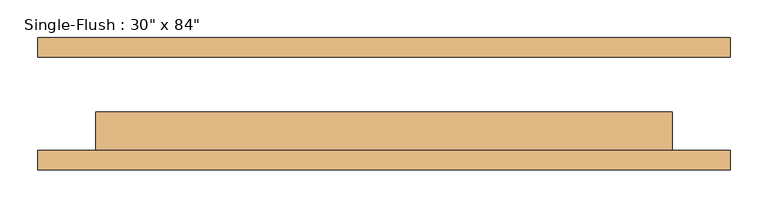
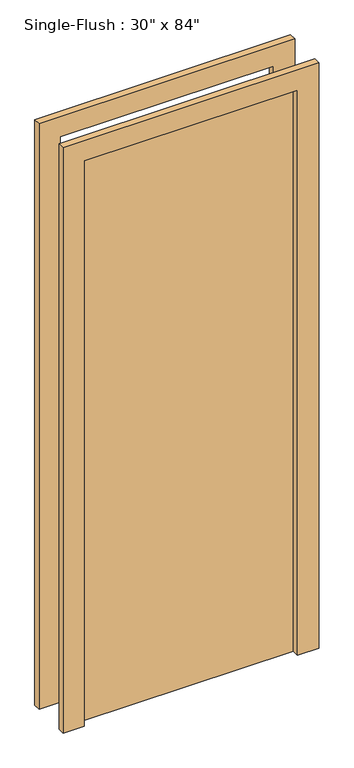
"""IFC4 building model written with IfcOpenShell, lengths in millimetres: door geometry."""

import ifcopenshell
import ifcopenshell.guid

model = None  # the IFC model being written
_history = None  # IfcOwnerHistory: only IFC2X3 demands one
_inside = {}  # id of a spatial element -> (the spatial element, [elements in it])
_under = {}  # id of a project, library or spatial element -> (it, [spatial elements below it])
_declared = {}  # id of a project -> (the project, [libraries it declares])
_typed = {}  # id of a type object -> (the type object, [elements of that type])
_made_of = {}  # id of a material, layer set ... -> (it, [elements and type objects made of it])


def new_model(schema):
    """Start an empty IFC model of exactly this schema.

    Asked for "IFC4X3", IfcOpenShell would pick the latest addendum, in which some entities
    have other attributes; the version numbers below select the first issue.
    IFC2X3 requires an IfcOwnerHistory on every rooted entity: one is made here for all.
    """
    global model, _history
    if schema == "IFC4X3":
        model = ifcopenshell.file(schema_version=(4, 3, 0, 0))
    else:
        model = ifcopenshell.file(schema=schema)
    _inside.clear()
    _under.clear()
    _declared.clear()
    _typed.clear()
    _made_of.clear()
    _history = None
    if model.schema == "IFC2X3":
        org = make("IfcOrganization", Name="unknown")
        user = make(
            "IfcPersonAndOrganization",
            ThePerson=make("IfcPerson", FamilyName="unknown"),
            TheOrganization=org,
        )
        app = make(
            "IfcApplication",
            ApplicationDeveloper=org,
            Version="unknown",
            ApplicationFullName="unknown",
            ApplicationIdentifier="unknown",
        )
        _history = make(
            "IfcOwnerHistory",
            OwningUser=user,
            OwningApplication=app,
            ChangeAction="ADDED",
            CreationDate=0,
        )
    return model


def make(cls, **values):
    """One entity of the class cls with the attributes given. An attribute that is None is left unset."""
    return model.create_entity(
        cls, **{name: value for name, value in values.items() if value is not None}
    )


def rooted(cls, **values):
    """An entity with a GlobalId (a new one), such as an element, a storey or a relation."""
    return make(cls, GlobalId=ifcopenshell.guid.new(), OwnerHistory=_history, **values)


def si_unit(unit_type, name, prefix=None):
    """IfcSIUnit, for example si_unit("LENGTHUNIT", "METRE", prefix="MILLI")."""
    return make("IfcSIUnit", UnitType=unit_type, Prefix=prefix, Name=name)


def assignment(units):
    """IfcUnitAssignment: the units of a project."""
    return None if units is None else make("IfcUnitAssignment", Units=units)


def point(xyz):
    """IfcCartesianPoint."""
    return None if xyz is None else make("IfcCartesianPoint", Coordinates=xyz)


def direction(xyz):
    """IfcDirection."""
    return None if xyz is None else make("IfcDirection", DirectionRatios=xyz)


def frame(location, z_axis=None, x_axis=None):
    """IfcAxis2Placement3D, a coordinate frame: its origin and axes. An axis left out is left unset."""
    return make(
        "IfcAxis2Placement3D",
        Location=point(location),
        Axis=direction(z_axis),
        RefDirection=direction(x_axis),
    )


def origin():
    """The frame at (0, 0, 0) with its axes left unset."""
    return frame((0.0, 0.0, 0.0))


def origin_with_axes():
    """The frame at (0, 0, 0) with the z axis (0, 0, 1) and the x axis (1, 0, 0) written out."""
    return frame((0.0, 0.0, 0.0), z_axis=(0.0, 0.0, 1.0), x_axis=(1.0, 0.0, 0.0))


def place(relative_to, where):
    """IfcLocalPlacement: puts the frame where relative to a parent placement (None: the world)."""
    return make(
        "IfcLocalPlacement", PlacementRelTo=relative_to, RelativePlacement=where
    )


def context(
    kind, dimensions, precision=None, world=None, true_north=None, identifier=None
):
    """IfcGeometricRepresentationContext, for example the 3D "Model" context."""
    return make(
        "IfcGeometricRepresentationContext",
        ContextIdentifier=identifier,
        ContextType=kind,
        CoordinateSpaceDimension=dimensions,
        Precision=precision,
        WorldCoordinateSystem=world,
        TrueNorth=true_north,
    )


def project(units=None, contexts=None):
    """IfcProject with its units and contexts."""
    return rooted(
        "IfcProject",
        Name="project",
        RepresentationContexts=contexts,
        UnitsInContext=assignment(units),
    )


def spatial(cls, under=None, at=None, **own):
    """A site, building, storey or space (cls), placed at a placement, below another one or the project."""
    s = rooted(cls, ObjectPlacement=at, **own)
    if under is not None:
        _under.setdefault(under.id(), (under, []))[1].append(s)
    return s


def polyline(points):
    """IfcPolyline through the points."""
    return make("IfcPolyline", Points=[point(p) for p in points])


def outline(outer, holes=None, kind="AREA"):
    """IfcArbitraryClosedProfileDef: a profile drawn as a closed curve; with holes, ...WithVoids."""
    if holes is None:
        return make("IfcArbitraryClosedProfileDef", ProfileType=kind, OuterCurve=outer)
    return make(
        "IfcArbitraryProfileDefWithVoids",
        ProfileType=kind,
        OuterCurve=outer,
        InnerCurves=holes,
    )


def extrude(swept, where, along, depth):
    """IfcExtrudedAreaSolid: the profile swept, set in the frame where, extruded along a direction by depth."""
    return make(
        "IfcExtrudedAreaSolid",
        SweptArea=swept,
        Position=where,
        ExtrudedDirection=direction(along),
        Depth=depth,
    )


def shape(context_of_items, identifier, shape_type, items):
    """IfcShapeRepresentation: the items that make up one representation, for example the "Body"."""
    return make(
        "IfcShapeRepresentation",
        ContextOfItems=context_of_items,
        RepresentationIdentifier=identifier,
        RepresentationType=shape_type,
        Items=items,
    )


def source(mapping_origin, context_of_items, identifier, shape_type, items):
    """IfcRepresentationMap: a shape defined once, which mapped items show again and again."""
    return make(
        "IfcRepresentationMap",
        MappingOrigin=mapping_origin,
        MappedRepresentation=shape(context_of_items, identifier, shape_type, items),
    )


def transform(
    local_origin,
    x_axis=None,
    y_axis=None,
    z_axis=None,
    scale=None,
    scale2=None,
    scale3=None,
    uniform=True,
):
    """IfcCartesianTransformationOperator3D, or its non-uniform kind. x_axis, y_axis, z_axis: its Axis1, 2, 3."""
    if uniform:
        return make(
            "IfcCartesianTransformationOperator3D",
            Axis1=direction(x_axis),
            Axis2=direction(y_axis),
            LocalOrigin=point(local_origin),
            Scale=scale,
            Axis3=direction(z_axis),
        )
    return make(
        "IfcCartesianTransformationOperator3DnonUniform",
        Axis1=direction(x_axis),
        Axis2=direction(y_axis),
        LocalOrigin=point(local_origin),
        Scale=scale,
        Axis3=direction(z_axis),
        Scale2=scale2,
        Scale3=scale3,
    )


def mapped(mapping_source, mapping_target):
    """IfcMappedItem: shows the shape of a source again, moved by a transform."""
    return make(
        "IfcMappedItem", MappingSource=mapping_source, MappingTarget=mapping_target
    )


def made_of(thing, what):
    """Note that an element or type object is made of a material, layer set ...; save() writes the relation."""
    if what is not None:
        _made_of.setdefault(what.id(), (what, []))[1].append(thing)
    return thing


def element(
    cls,
    number,
    at=None,
    inside=None,
    cuts=None,
    type_object=None,
    material=None,
    context=None,
    identifier="Body",
    shape_type=None,
    held_by="IfcProductDefinitionShape",
    body=None,
    shapes=None,
    **own,
):
    """One element of the class cls, such as IfcWall. Its Tag is "e" and its number.

    at: its placement. inside: the storey or other place that contains it. cuts: it is an
    opening in that element (IfcRelVoidsElement). A single representation is given by context,
    identifier, shape_type and body (its items); several are given by shapes. held_by: the class
    of the entity that holds the representations. save() writes the other relations.
    """
    e = rooted(cls, Tag="e%d" % number, ObjectPlacement=at, **own)
    if body is not None:
        shapes = [shape(context, identifier, shape_type, body)]
    if shapes is not None:
        e.Representation = make(held_by, Representations=shapes)
    if inside is not None:
        _inside.setdefault(inside.id(), (inside, []))[1].append(e)
    if cuts is not None:
        rooted(
            "IfcRelVoidsElement", RelatingBuildingElement=cuts, RelatedOpeningElement=e
        )
    if type_object is not None:
        _typed.setdefault(type_object.id(), (type_object, []))[1].append(e)
    return made_of(e, material)


def aggregate(whole, parts):
    """IfcRelAggregates: a whole, such as a stair, and the parts it consists of."""
    return rooted("IfcRelAggregates", RelatingObject=whole, RelatedObjects=parts)


def save(model, path):
    """Write the relations noted so far, then the file.

    IfcRelAggregates (storeys below a building ...), IfcRelContainedInSpatialStructure (elements
    in a storey), IfcRelDefinesByType, IfcRelAssociatesMaterial and IfcRelDeclares: one each for
    every whole, place, type object, material and project.
    """
    for whole, parts in _under.values():
        aggregate(whole, parts)
    for where, things in _inside.values():
        rooted(
            "IfcRelContainedInSpatialStructure",
            RelatedElements=things,
            RelatingStructure=where,
        )
    for kind, things in _typed.values():
        rooted("IfcRelDefinesByType", RelatedObjects=things, RelatingType=kind)
    for what, things in _made_of.values():
        rooted("IfcRelAssociatesMaterial", RelatedObjects=things, RelatingMaterial=what)
    for by, libraries in _declared.values():
        rooted("IfcRelDeclares", RelatingContext=by, RelatedDefinitions=libraries)
    model.write(path)


def door_702a1063(model_context):
    return source(origin(), model_context, "Body", "SweptSolid", [
        extrude(outline(polyline([(2209.8, -457.2), (0.0, -457.2), (0.0, -381.0), (2133.6, -381.0), (2133.6, 381.0), (0.0, 381.0), (0.0, 457.2), (2209.8, 457.2), (2209.8, -457.2)])), frame((0.0, -87.3125, 0.0), z_axis=(0.0, 1.0, 0.0), x_axis=(0.0, 0.0, 1.0)), (0.0, 0.0, 1.0), 25.4),
        extrude(outline(polyline([(2209.8, 457.2), (2209.8, -457.2), (0.0, -457.2), (0.0, -381.0), (2133.6, -381.0), (2133.6, 381.0), (0.0, 381.0), (0.0, 457.2), (2209.8, 457.2)])), frame((0.0, 61.9125, 0.0), z_axis=(0.0, 1.0, 0.0), x_axis=(0.0, 0.0, 1.0)), (0.0, 0.0, 1.0), 25.4),
        extrude(outline(polyline([(381.0, -11.1125), (381.0, -61.9125), (-381.0, -61.9125), (-381.0, -11.1125), (381.0, -11.1125)])), origin_with_axes(), (0.0, 0.0, 1.0), 2133.6),
    ])


if __name__ == "__main__":
    model = new_model("IFC4")
    model_context = context("Model", 3, world=origin())
    ifc_project = project(units=[si_unit("LENGTHUNIT", "METRE", prefix="MILLI")], contexts=[model_context])
    site = spatial("IfcSite", under=ifc_project)
    building = spatial("IfcBuilding", under=site)
    placement = place(None, origin())
    door_shape = door_702a1063(model_context)
    element("IfcDoor", 1, ObjectType="Single-Flush : 30\" x 84\"", at=placement, inside=building, context=model_context, shape_type="MappedRepresentation", body=[
        mapped(door_shape, transform((0.0, 0.0, 0.0), x_axis=(1.0, 0.0, 0.0), y_axis=(0.0, 1.0, 0.0), z_axis=(0.0, 0.0, 1.0))),
    ])
    save(model, "model.ifc")

# Revit data of these elements
# Type "Single-Flush : 30\" x 84\""
#   Type Mark = "46"
#   Assembly Code = "C1020"
#   Thickness = 0' - 2"
#   Height = 7' - 0"
#   Trim Projection Ext = 0' - 1"
#   Trim Projection Int = 0' - 1"
#   Trim Width = 0' - 3"
#   Width = 2' - 6"
#   Door Material = none
#   Frame Material = none
#   Function = (empty or 0)
#   Wall Closure = (empty or 0)
